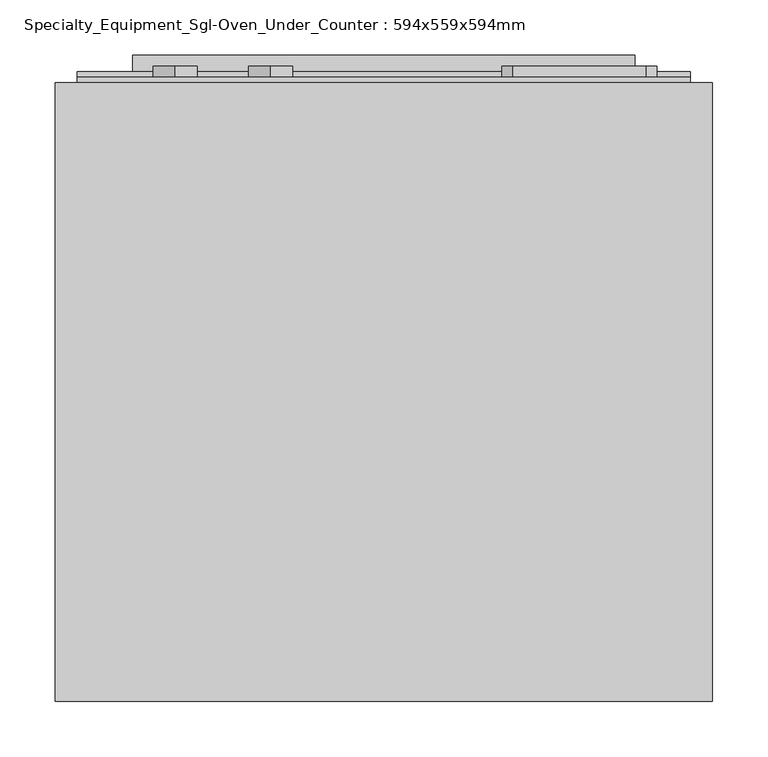
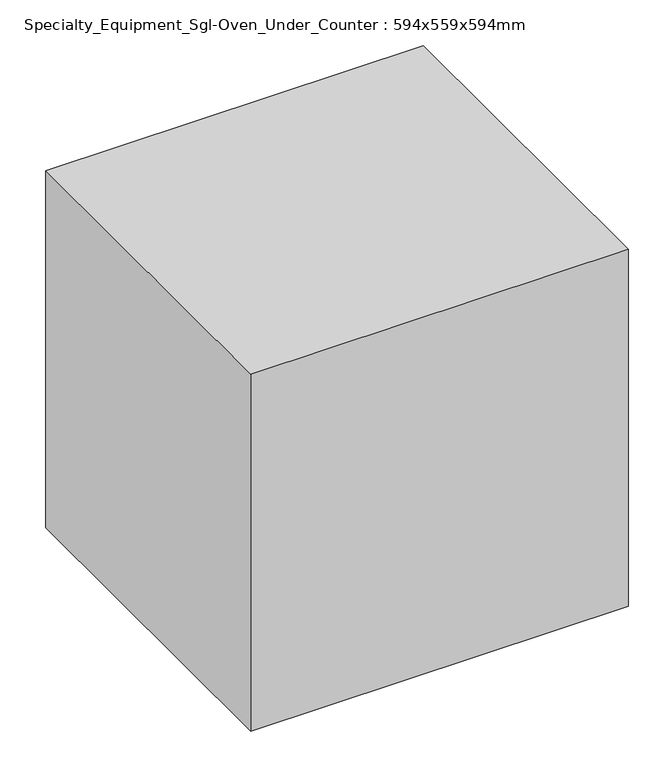
"""IFC4 building model written with IfcOpenShell, lengths in millimetres: proxy geometry, Specialty_Equipment_Sgl-Oven_Under_Counter : 594x559x594mm."""

import ifcopenshell
import ifcopenshell.guid

model = None  # the IFC model being written
_history = None  # IfcOwnerHistory: only IFC2X3 demands one
_inside = {}  # id of a spatial element -> (the spatial element, [elements in it])
_under = {}  # id of a project, library or spatial element -> (it, [spatial elements below it])
_declared = {}  # id of a project -> (the project, [libraries it declares])
_typed = {}  # id of a type object -> (the type object, [elements of that type])
_made_of = {}  # id of a material, layer set ... -> (it, [elements and type objects made of it])


def new_model(schema):
    """Start an empty IFC model of exactly this schema.

    Asked for "IFC4X3", IfcOpenShell would pick the latest addendum, in which some entities
    have other attributes; the version numbers below select the first issue.
    IFC2X3 requires an IfcOwnerHistory on every rooted entity: one is made here for all.
    """
    global model, _history
    if schema == "IFC4X3":
        model = ifcopenshell.file(schema_version=(4, 3, 0, 0))
    else:
        model = ifcopenshell.file(schema=schema)
    _inside.clear()
    _under.clear()
    _declared.clear()
    _typed.clear()
    _made_of.clear()
    _history = None
    if model.schema == "IFC2X3":
        org = make("IfcOrganization", Name="unknown")
        user = make(
            "IfcPersonAndOrganization",
            ThePerson=make("IfcPerson", FamilyName="unknown"),
            TheOrganization=org,
        )
        app = make(
            "IfcApplication",
            ApplicationDeveloper=org,
            Version="unknown",
            ApplicationFullName="unknown",
            ApplicationIdentifier="unknown",
        )
        _history = make(
            "IfcOwnerHistory",
            OwningUser=user,
            OwningApplication=app,
            ChangeAction="ADDED",
            CreationDate=0,
        )
    return model


def make(cls, **values):
    """One entity of the class cls with the attributes given. An attribute that is None is left unset."""
    return model.create_entity(
        cls, **{name: value for name, value in values.items() if value is not None}
    )


def rooted(cls, **values):
    """An entity with a GlobalId (a new one), such as an element, a storey or a relation."""
    return make(cls, GlobalId=ifcopenshell.guid.new(), OwnerHistory=_history, **values)


def si_unit(unit_type, name, prefix=None):
    """IfcSIUnit, for example si_unit("LENGTHUNIT", "METRE", prefix="MILLI")."""
    return make("IfcSIUnit", UnitType=unit_type, Prefix=prefix, Name=name)


def assignment(units):
    """IfcUnitAssignment: the units of a project."""
    return None if units is None else make("IfcUnitAssignment", Units=units)


def point(xyz):
    """IfcCartesianPoint."""
    return None if xyz is None else make("IfcCartesianPoint", Coordinates=xyz)


def direction(xyz):
    """IfcDirection."""
    return None if xyz is None else make("IfcDirection", DirectionRatios=xyz)


def frame(location, z_axis=None, x_axis=None):
    """IfcAxis2Placement3D, a coordinate frame: its origin and axes. An axis left out is left unset."""
    return make(
        "IfcAxis2Placement3D",
        Location=point(location),
        Axis=direction(z_axis),
        RefDirection=direction(x_axis),
    )


def frame_2d(location, x_axis=None):
    """IfcAxis2Placement2D, a coordinate frame in the plane: its origin and x axis."""
    return make(
        "IfcAxis2Placement2D", Location=point(location), RefDirection=direction(x_axis)
    )


def origin():
    """The frame at (0, 0, 0) with its axes left unset."""
    return frame((0.0, 0.0, 0.0))


def place(relative_to, where):
    """IfcLocalPlacement: puts the frame where relative to a parent placement (None: the world)."""
    return make(
        "IfcLocalPlacement", PlacementRelTo=relative_to, RelativePlacement=where
    )


def context(
    kind, dimensions, precision=None, world=None, true_north=None, identifier=None
):
    """IfcGeometricRepresentationContext, for example the 3D "Model" context."""
    return make(
        "IfcGeometricRepresentationContext",
        ContextIdentifier=identifier,
        ContextType=kind,
        CoordinateSpaceDimension=dimensions,
        Precision=precision,
        WorldCoordinateSystem=world,
        TrueNorth=true_north,
    )


def project(units=None, contexts=None):
    """IfcProject with its units and contexts."""
    return rooted(
        "IfcProject",
        Name="project",
        RepresentationContexts=contexts,
        UnitsInContext=assignment(units),
    )


def spatial(cls, under=None, at=None, **own):
    """A site, building, storey or space (cls), placed at a placement, below another one or the project."""
    s = rooted(cls, ObjectPlacement=at, **own)
    if under is not None:
        _under.setdefault(under.id(), (under, []))[1].append(s)
    return s


def polyline(points):
    """IfcPolyline through the points."""
    return make("IfcPolyline", Points=[point(p) for p in points])


def circle_curve(where, radius):
    """IfcCircle in the frame where."""
    return make("IfcCircle", Position=where, Radius=radius)


def trimmed(basis, trim1, trim2, sense, master):
    """IfcTrimmedCurve: the piece of a basis curve between two trims."""
    return make(
        "IfcTrimmedCurve",
        BasisCurve=basis,
        Trim1=trim1,
        Trim2=trim2,
        SenseAgreement=sense,
        MasterRepresentation=master,
    )


def segment(curve, same_sense, transition):
    """IfcCompositeCurveSegment."""
    return make(
        "IfcCompositeCurveSegment",
        Transition=transition,
        SameSense=same_sense,
        ParentCurve=curve,
    )


def composite_curve(segments, self_intersect=None):
    """IfcCompositeCurve: segments joined end to end."""
    return make("IfcCompositeCurve", Segments=segments, SelfIntersect=self_intersect)


def outline(outer, holes=None, kind="AREA"):
    """IfcArbitraryClosedProfileDef: a profile drawn as a closed curve; with holes, ...WithVoids."""
    if holes is None:
        return make("IfcArbitraryClosedProfileDef", ProfileType=kind, OuterCurve=outer)
    return make(
        "IfcArbitraryProfileDefWithVoids",
        ProfileType=kind,
        OuterCurve=outer,
        InnerCurves=holes,
    )


def extrude(swept, where, along, depth):
    """IfcExtrudedAreaSolid: the profile swept, set in the frame where, extruded along a direction by depth."""
    return make(
        "IfcExtrudedAreaSolid",
        SweptArea=swept,
        Position=where,
        ExtrudedDirection=direction(along),
        Depth=depth,
    )


def faces_of(points, faces, orient=None, outer=None):
    """IfcFace entities. A face is a list of loops; a loop is a list of indices into points, from 0.

    orient and outer hold one flag for each loop. By default every Orientation is true, the
    first loop of a face is its IfcFaceOuterBound and the others are IfcFaceBound.
    """
    made = []
    for i, loops in enumerate(faces):
        bounds = []
        for j, loop in enumerate(loops):
            is_outer = j == 0 if outer is None else outer[i][j]
            bounds.append(
                make(
                    "IfcFaceOuterBound" if is_outer else "IfcFaceBound",
                    Bound=make("IfcPolyLoop", Polygon=[points[k] for k in loop]),
                    Orientation=True if orient is None else orient[i][j],
                )
            )
        made.append(make("IfcFace", Bounds=bounds))
    return made


def faceted_brep(points, faces, orient=None, outer=None, voids=None):
    """IfcFacetedBrep: a solid bounded by flat faces; with voids (closed shells), ...WithVoids."""
    shared = [point(p) for p in points]
    hull = make("IfcClosedShell", CfsFaces=faces_of(shared, faces, orient, outer))
    if voids is None:
        return make("IfcFacetedBrep", Outer=hull)
    return make(
        "IfcFacetedBrepWithVoids",
        Outer=hull,
        Voids=[
            make(cls, CfsFaces=faces_of(shared, fs, o, b)) for cls, fs, o, b in voids
        ],
    )


def shape(context_of_items, identifier, shape_type, items):
    """IfcShapeRepresentation: the items that make up one representation, for example the "Body"."""
    return make(
        "IfcShapeRepresentation",
        ContextOfItems=context_of_items,
        RepresentationIdentifier=identifier,
        RepresentationType=shape_type,
        Items=items,
    )


def source(mapping_origin, context_of_items, identifier, shape_type, items):
    """IfcRepresentationMap: a shape defined once, which mapped items show again and again."""
    return make(
        "IfcRepresentationMap",
        MappingOrigin=mapping_origin,
        MappedRepresentation=shape(context_of_items, identifier, shape_type, items),
    )


def transform(
    local_origin,
    x_axis=None,
    y_axis=None,
    z_axis=None,
    scale=None,
    scale2=None,
    scale3=None,
    uniform=True,
):
    """IfcCartesianTransformationOperator3D, or its non-uniform kind. x_axis, y_axis, z_axis: its Axis1, 2, 3."""
    if uniform:
        return make(
            "IfcCartesianTransformationOperator3D",
            Axis1=direction(x_axis),
            Axis2=direction(y_axis),
            LocalOrigin=point(local_origin),
            Scale=scale,
            Axis3=direction(z_axis),
        )
    return make(
        "IfcCartesianTransformationOperator3DnonUniform",
        Axis1=direction(x_axis),
        Axis2=direction(y_axis),
        LocalOrigin=point(local_origin),
        Scale=scale,
        Axis3=direction(z_axis),
        Scale2=scale2,
        Scale3=scale3,
    )


def mapped(mapping_source, mapping_target):
    """IfcMappedItem: shows the shape of a source again, moved by a transform."""
    return make(
        "IfcMappedItem", MappingSource=mapping_source, MappingTarget=mapping_target
    )


def made_of(thing, what):
    """Note that an element or type object is made of a material, layer set ...; save() writes the relation."""
    if what is not None:
        _made_of.setdefault(what.id(), (what, []))[1].append(thing)
    return thing


def element(
    cls,
    number,
    at=None,
    inside=None,
    cuts=None,
    type_object=None,
    material=None,
    context=None,
    identifier="Body",
    shape_type=None,
    held_by="IfcProductDefinitionShape",
    body=None,
    shapes=None,
    **own,
):
    """One element of the class cls, such as IfcWall. Its Tag is "e" and its number.

    at: its placement. inside: the storey or other place that contains it. cuts: it is an
    opening in that element (IfcRelVoidsElement). A single representation is given by context,
    identifier, shape_type and body (its items); several are given by shapes. held_by: the class
    of the entity that holds the representations. save() writes the other relations.
    """
    e = rooted(cls, Tag="e%d" % number, ObjectPlacement=at, **own)
    if body is not None:
        shapes = [shape(context, identifier, shape_type, body)]
    if shapes is not None:
        e.Representation = make(held_by, Representations=shapes)
    if inside is not None:
        _inside.setdefault(inside.id(), (inside, []))[1].append(e)
    if cuts is not None:
        rooted(
            "IfcRelVoidsElement", RelatingBuildingElement=cuts, RelatedOpeningElement=e
        )
    if type_object is not None:
        _typed.setdefault(type_object.id(), (type_object, []))[1].append(e)
    return made_of(e, material)


def aggregate(whole, parts):
    """IfcRelAggregates: a whole, such as a stair, and the parts it consists of."""
    return rooted("IfcRelAggregates", RelatingObject=whole, RelatedObjects=parts)


def save(model, path):
    """Write the relations noted so far, then the file.

    IfcRelAggregates (storeys below a building ...), IfcRelContainedInSpatialStructure (elements
    in a storey), IfcRelDefinesByType, IfcRelAssociatesMaterial and IfcRelDeclares: one each for
    every whole, place, type object, material and project.
    """
    for whole, parts in _under.values():
        aggregate(whole, parts)
    for where, things in _inside.values():
        rooted(
            "IfcRelContainedInSpatialStructure",
            RelatedElements=things,
            RelatingStructure=where,
        )
    for kind, things in _typed.values():
        rooted("IfcRelDefinesByType", RelatedObjects=things, RelatingType=kind)
    for what, things in _made_of.values():
        rooted("IfcRelAssociatesMaterial", RelatedObjects=things, RelatingMaterial=what)
    for by, libraries in _declared.values():
        rooted("IfcRelDeclares", RelatingContext=by, RelatedDefinitions=libraries)
    model.write(path)


def specialty_equipment_sgl_oven_under_counter_594x559x594mm_8b8b962d(model_context):
    return source(origin(), model_context, "Body", "SolidModel", [
        faceted_brep([(266.0578446, 665.0, 860.0), (-327.9421554, 665.0, 860.0), (-327.9421554, 106.0, 860.0), (266.0578446, 106.0, 860.0), (266.0578446, 665.0, 266.0), (266.0578446, 106.0, 266.0), (-327.9421554, 106.0, 266.0), (-327.9421554, 665.0, 266.0), (246.0578446, 665.0, 740.4988468), (-307.9421554, 665.0, 740.4988468), (-307.9421554, 665.0, 286.0), (246.0578446, 665.0, 286.0), (246.0578446, 181.9875773, 740.4988468), (246.0578446, 181.9875773, 286.0), (-307.9421554, 181.9875773, 286.0), (-307.9421554, 181.9875773, 740.4988468)], [[[0, 1, 2, 3]], [[4, 5, 6, 7]], [[1, 0, 4, 7], [8, 9, 10, 11]], [[2, 1, 7, 6]], [[3, 2, 6, 5]], [[0, 3, 5, 4]], [[12, 13, 14, 15]], [[12, 15, 9, 8]], [[15, 14, 10, 9]], [[14, 13, 11, 10]], [[13, 12, 8, 11]]]),
        extrude(outline(polyline([(-307.9421554, 670.0), (246.0578446, 670.0), (246.0578446, 665.0), (-307.9421554, 665.0), (-307.9421554, 670.0)])), frame((0.0, 0.0, 740.4988468), z_axis=(0.0, 0.0, 1.0), x_axis=(1.0, 0.0, 0.0)), (0.0, 0.0, 1.0), 99.5011532),
        extrude(outline(polyline([(86.0578446, 680.0), (206.0578446, 680.0), (206.0578446, 665.0), (86.0578446, 665.0), (86.0578446, 680.0)])), frame((0.0, 0.0, 790.4988468), z_axis=(0.0, 0.0, 1.0), x_axis=(1.0, 0.0, 0.0)), (0.0, 0.0, 1.0), 28.8192733),
        extrude(outline(composite_curve([segment(trimmed(circle_curve(frame_2d((785.4988468, -219.501226)), 20.0), [point((805.4988468, -219.501226))], [point((765.4988468, -219.501226))], False, "CARTESIAN"), True, "CONTINUOUS"), segment(trimmed(circle_curve(frame_2d((785.4988468, -219.501226)), 20.0), [point((765.4988468, -219.501226))], [point((805.4988468, -219.501226))], False, "CARTESIAN"), True, "CONTINUOUS")], self_intersect=False)), frame((0.0, 665.0, 0.0), z_axis=(0.0, 1.0, 0.0), x_axis=(0.0, 0.0, 1.0)), (0.0, 0.0, 1.0), 15.0),
        extrude(outline(composite_curve([segment(trimmed(circle_curve(frame_2d((785.4988468, -133.1879639)), 20.0), [point((805.4988468, -133.1879639))], [point((765.4988468, -133.1879639))], False, "CARTESIAN"), True, "CONTINUOUS"), segment(trimmed(circle_curve(frame_2d((785.4988468, -133.1879639)), 20.0), [point((765.4988468, -133.1879639))], [point((805.4988468, -133.1879639))], False, "CARTESIAN"), True, "CONTINUOUS")], self_intersect=False)), frame((0.0, 665.0, 0.0), z_axis=(0.0, 1.0, 0.0), x_axis=(0.0, 0.0, 1.0)), (0.0, 0.0, 1.0), 15.0),
        extrude(outline(composite_curve([segment(trimmed(circle_curve(frame_2d((770.4988468, 86.0578446)), 10.0), [point((780.4988468, 86.0578446))], [point((760.4988468, 86.0578446))], False, "CARTESIAN"), True, "CONTINUOUS"), segment(trimmed(circle_curve(frame_2d((770.4988468, 86.0578446)), 10.0), [point((760.4988468, 86.0578446))], [point((780.4988468, 86.0578446))], False, "CARTESIAN"), True, "CONTINUOUS")], self_intersect=False)), frame((0.0, 665.0, 0.0), z_axis=(0.0, 1.0, 0.0), x_axis=(0.0, 0.0, 1.0)), (0.0, 0.0, 1.0), 15.0),
        extrude(outline(composite_curve([segment(trimmed(circle_curve(frame_2d((770.4988468, 116.0578446)), 10.0), [point((780.4988468, 116.0578446))], [point((760.4988468, 116.0578446))], False, "CARTESIAN"), True, "CONTINUOUS"), segment(trimmed(circle_curve(frame_2d((770.4988468, 116.0578446)), 10.0), [point((760.4988468, 116.0578446))], [point((780.4988468, 116.0578446))], False, "CARTESIAN"), True, "CONTINUOUS")], self_intersect=False)), frame((0.0, 665.0, 0.0), z_axis=(0.0, 1.0, 0.0), x_axis=(0.0, 0.0, 1.0)), (0.0, 0.0, 1.0), 15.0),
        extrude(outline(composite_curve([segment(trimmed(circle_curve(frame_2d((770.4988468, 146.0578446)), 10.0), [point((780.4988468, 146.0578446))], [point((760.4988468, 146.0578446))], False, "CARTESIAN"), True, "CONTINUOUS"), segment(trimmed(circle_curve(frame_2d((770.4988468, 146.0578446)), 10.0), [point((760.4988468, 146.0578446))], [point((780.4988468, 146.0578446))], False, "CARTESIAN"), True, "CONTINUOUS")], self_intersect=False)), frame((0.0, 665.0, 0.0), z_axis=(0.0, 1.0, 0.0), x_axis=(0.0, 0.0, 1.0)), (0.0, 0.0, 1.0), 15.0),
        extrude(outline(composite_curve([segment(trimmed(circle_curve(frame_2d((770.4988468, 176.0578446)), 10.0), [point((780.4988468, 176.0578446))], [point((760.4988468, 176.0578446))], False, "CARTESIAN"), True, "CONTINUOUS"), segment(trimmed(circle_curve(frame_2d((770.4988468, 176.0578446)), 10.0), [point((760.4988468, 176.0578446))], [point((780.4988468, 176.0578446))], False, "CARTESIAN"), True, "CONTINUOUS")], self_intersect=False)), frame((0.0, 665.0, 0.0), z_axis=(0.0, 1.0, 0.0), x_axis=(0.0, 0.0, 1.0)), (0.0, 0.0, 1.0), 15.0),
        extrude(outline(composite_curve([segment(trimmed(circle_curve(frame_2d((770.4988468, 206.0578446)), 10.0), [point((780.4988468, 206.0578446))], [point((760.4988468, 206.0578446))], False, "CARTESIAN"), True, "CONTINUOUS"), segment(trimmed(circle_curve(frame_2d((770.4988468, 206.0578446)), 10.0), [point((760.4988468, 206.0578446))], [point((780.4988468, 206.0578446))], False, "CARTESIAN"), True, "CONTINUOUS")], self_intersect=False)), frame((0.0, 665.0, 0.0), z_axis=(0.0, 1.0, 0.0), x_axis=(0.0, 0.0, 1.0)), (0.0, 0.0, 1.0), 15.0),
        extrude(outline(polyline([(-257.9421554, 690.0), (196.0578446, 690.0), (196.0578446, 675.0), (-257.9421554, 675.0), (-257.9421554, 690.0)])), frame((0.0, 0.0, 697.6588468), z_axis=(0.0, 0.0, 1.0), x_axis=(1.0, 0.0, 0.0)), (0.0, 0.0, 1.0), 20.0),
        extrude(outline(polyline([(286.0, -307.9421554), (286.0, 246.0578446), (740.4988468, 246.0578446), (740.4988468, -307.9421554), (286.0, -307.9421554)]), holes=[polyline([(336.0, -267.9421554), (667.6588468, -267.9421554), (667.6588468, 206.0578446), (336.0, 206.0578446), (336.0, -267.9421554)])]), frame((0.0, 665.0, 0.0), z_axis=(0.0, 1.0, 0.0), x_axis=(0.0, 0.0, 1.0)), (0.0, 0.0, 1.0), 10.0),
    ])


if __name__ == "__main__":
    model = new_model("IFC4")
    model_context = context("Model", 3, world=origin())
    ifc_project = project(units=[si_unit("LENGTHUNIT", "METRE", prefix="MILLI")], contexts=[model_context])
    site = spatial("IfcSite", under=ifc_project)
    building = spatial("IfcBuilding", under=site)
    placement = place(None, origin())
    specialty_equipment_sgl_oven_under_counter_594x559x594mm_shape = specialty_equipment_sgl_oven_under_counter_594x559x594mm_8b8b962d(model_context)
    element("IfcBuildingElementProxy", 1, Name="Specialty_Equipment_Sgl-Oven_Under_Counter : 594x559x594mm", ObjectType="Specialty_Equipment_Sgl-Oven_Under_Counter : 594x559x594mm", at=placement, inside=building, context=model_context, shape_type="MappedRepresentation", body=[
        mapped(specialty_equipment_sgl_oven_under_counter_594x559x594mm_shape, transform((0.0, 0.0, 0.0), x_axis=(1.0, 0.0, 0.0), y_axis=(0.0, 1.0, 0.0), z_axis=(0.0, 0.0, 1.0))),
    ])
    save(model, "model.ifc")

# Revit data of these elements
# Type "Specialty_Equipment_Sgl-Oven_Under_Counter : 594x559x594mm"
#   Label = "OVEN"
#   Keynote = "N"
#   Depth = 559 mm
#   Height = 594 mm
#   Placement Hgt = 266 mm
#   Width = 594 mm
#   Oven Material = Metal - Stainless Steel
#   Default Elevation = 0
# Element 1 (IfcBuildingElementProxy, "Specialty_Equipment_Sgl-Oven_Under_Counter : 594x559x594mm")
#   Materials on its faces: "Metal - Paint Finish - Dark Gray, Matte", "Metal - Stainless Steel", "Plastic - Black"
# Materials
#   "Metal - Stainless Steel": class "Metal", colour RGB 173 173 173, transparency 0
#   "Metal - Paint Finish - Dark Gray, Matte": class "Paint", colour RGB 98 98 98, transparency 0
#   "Plastic - Black": class "Plastic", colour RGB 0 0 0, transparency 0
